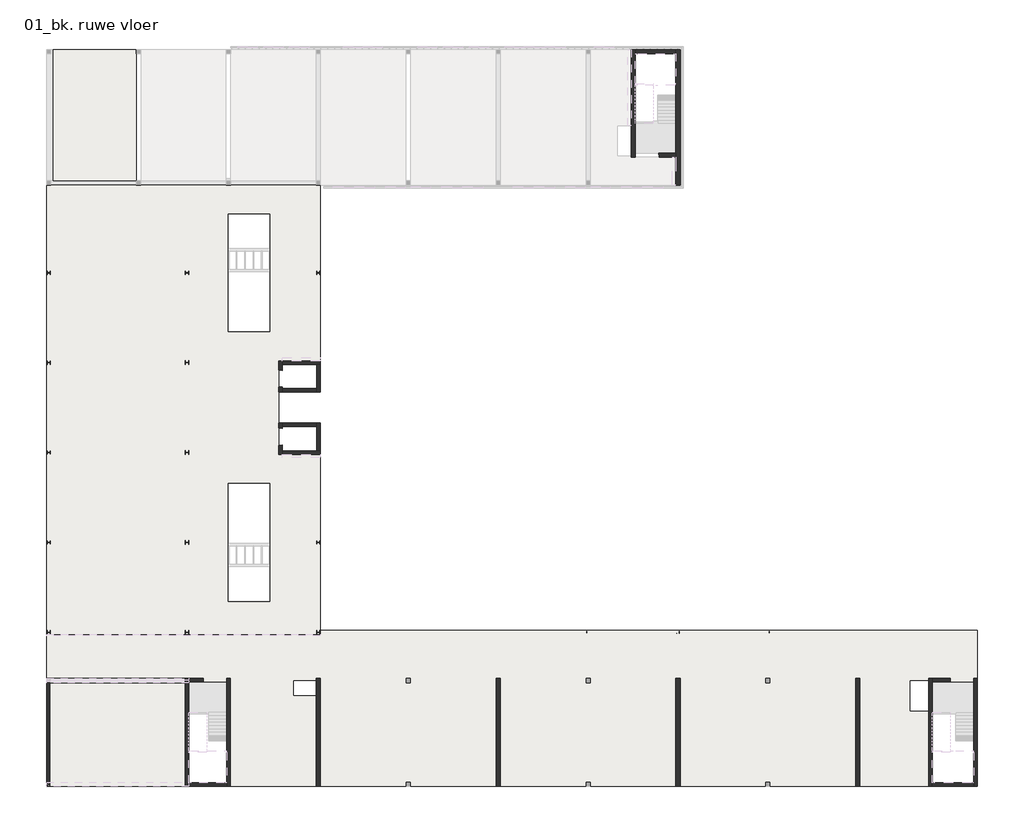
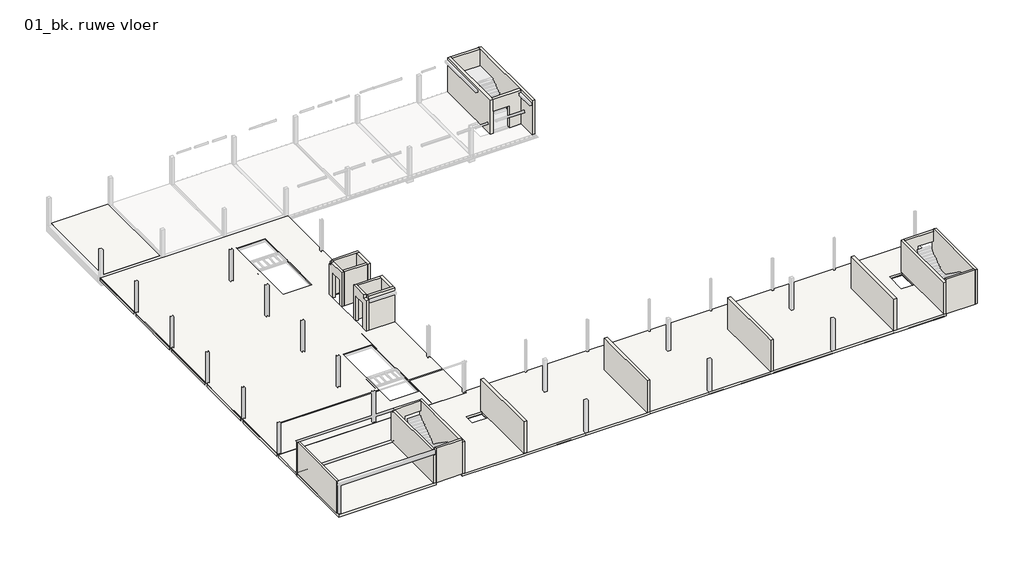
# One storey, part 1 of 4: 25 walls, 20 slabs.
# Revit data of these elements (continued)
# Element 13 (IfcSlab, "NLRS_23_FL_kanaalplaat 260_gen_rsf") (continued)
#   Phase Created = NLRS_nieuw
#   Materials on its faces: "NLRS_f2_beton prefab_gen_rsf"
# Element 14 (IfcSlab, "NLRS_23_FL_kanaalplaat 260_gen_rsf")
#   IfcGUID = "0OswKhMc1Dju7i6LqsCl1d"
#   built-in parameter 1001955 = -1.5708 (stored number, unit not read)
#   Height Offset From Level = -70 mm
#   built-in parameter 1001954 = 1
#   IsExternal = no
#   LoadBearing = yes
#   Phase Created = NLRS_nieuw
#   Materials on its faces: "NLRS_f2_beton prefab_gen_rsf"
# Element 15 (IfcSlab, "NLRS_23_FL_kanaalplaat 260_gen_rsf")
#   IfcGUID = "0OswKhMc1Dju7i6LqsCl1m"
#   Height Offset From Level = -70 mm
#   built-in parameter 1001954 = 1
#   IsExternal = no
#   LoadBearing = yes
#   Phase Created = NLRS_nieuw
#   Materials on its faces: "NLRS_f2_beton prefab_gen_rsf"
# Element 16 (IfcSlab, "NLRS_23_FL_kanaalplaat 260_gen_rsf")
#   IfcGUID = "0OswKhMc1Dju7i6LqsCl2B"
#   built-in parameter 1001955 = 1.5708 (stored number, unit not read)
#   Height Offset From Level = -70 mm
#   built-in parameter 1001954 = 1
#   IsExternal = no
#   LoadBearing = yes
#   Phase Created = NLRS_nieuw
#   Materials on its faces: "NLRS_f2_beton prefab_gen_rsf"
# Element 17 (IfcSlab, "NLRS_23_FL_breedplaat 260_gen_rsf")
#   IfcGUID = "3aMdMHoe12P9KDGPyaIhcT"
#   built-in parameter 1001955 = 1.5708 (stored number, unit not read)
#   Height Offset From Level = 0 mm
#   built-in parameter 1001954 = 1
#   IsExternal = no
#   LoadBearing = yes
#   Phase Created = NLRS_nieuw
#   Materials on its faces: "NLRS_f2_beton ihwg_gen_rsf"
# Element 18 (IfcSlab, "NLRS_23_FL_breedplaat schil 60_gen_rsf")
#   IfcGUID = "2hjDq_lp57$vrUvPCETdlA"
#   Comments = ""
#   built-in parameter 1001955 = -1.5708 (stored number, unit not read)
#   Height Offset From Level = -200 mm
#   built-in parameter 1001954 = 1
#   IsExternal = no
#   LoadBearing = yes
#   Phase Created = NLRS_nieuw
#   Materials on its faces: "NLRS_f2_beton prefab_gen_rsf"
# Element 19 (IfcSlab, "NLRS_23_FL_breedplaat schil 60_gen_rsf")
#   IfcGUID = "2hjDq_lp57$vrUvPCETOIZ"
#   Comments = ""
#   built-in parameter 1001955 = -1.5708 (stored number, unit not read)
#   Height Offset From Level = -200 mm
#   built-in parameter 1001954 = 1
#   IsExternal = no
#   LoadBearing = yes
#   Phase Created = NLRS_nieuw
#   Materials on its faces: "NLRS_f2_beton prefab_gen_rsf"
# Element 20 (IfcSlab, "NLRS_23_FL_breedplaat schil 60_gen_rsf")
#   IfcGUID = "1q3Kx8wcTFnf_3PJz4ij95"
#   Comments = ""
#   Height Offset From Level = -200 mm
#   built-in parameter 1001954 = 1
#   IsExternal = no
#   LoadBearing = yes
#   Phase Created = NLRS_nieuw
#   Materials on its faces: "NLRS_f2_beton prefab_gen_rsf"
# Element 21 (IfcWall, "NLRS_22_WA_beton ihw 250_gen_rsf")
#   IfcGUID = "13lTCcCQ95UOWcvnmPh7qn"
#   Comments = ""
#   Top Offset = 0 mm
#   Base Offset = 0 mm
#   wall height = 3540 mm
#   IsExternal = no
#   LoadBearing = yes
#   Phase Created = NLRS_nieuw
#   Base Constraint = 01_bk. ruwe vloer
#   Top Constraint = 02_ok ruwe vloer
#   Materials on its faces: "NLRS_f2_beton ihwg_gen_rsf"
# Element 22 (IfcWall, "NLRS_22_WA_beton ihw 250_gen_rsf")
#   IfcGUID = "13lTCcCQ95UOWcvnmPh7qi"
#   Comments = ""
#   Top Offset = 0 mm
#   Base Offset = 0 mm
#   wall height = 3540 mm
#   IsExternal = no
#   LoadBearing = yes
#   Phase Created = NLRS_nieuw
#   Base Constraint = 01_bk. ruwe vloer
#   Top Constraint = 02_ok ruwe vloer
#   Materials on its faces: "NLRS_f2_beton ihwg_gen_rsf"
# Element 23 (IfcWall, "NLRS_22_WA_beton ihw 300_gen_rsf")
#   IfcGUID = "13lTCcCQ95UOWcvnmPh7qk"
#   Comments = ""
#   Top Offset = 0 mm
#   Base Offset = 0 mm
#   wall height = 3540 mm
#   IsExternal = no
#   LoadBearing = yes
#   Phase Created = NLRS_nieuw
#   Base Constraint = 01_bk. ruwe vloer
#   Top Constraint = 02_ok ruwe vloer
#   Materials on its faces: "NLRS_f2_beton ihwg_gen_rsf"
# Element 24 (IfcWall, "NLRS_22_WA_beton ihw 300_gen_rsf")
#   IfcGUID = "13lTCcCQ95UOWcvnmPh7qg"
#   Comments = ""
#   Top Offset = 0 mm
#   Base Offset = 0 mm
#   wall height = 3540 mm
#   IsExternal = no
#   LoadBearing = yes
#   Phase Created = NLRS_nieuw
#   Base Constraint = 01_bk. ruwe vloer
#   Top Constraint = 02_ok ruwe vloer
#   Materials on its faces: "NLRS_f2_beton ihwg_gen_rsf"
# Element 25 (IfcWall, "NLRS_22_WA_beton ihw 300_gen_rsf")
#   IfcGUID = "13lTCcCQ95UOWcvnmPh7qc"
#   Comments = ""
#   Top Offset = 0 mm
#   Base Offset = 0 mm
#   wall height = 3540 mm
#   IsExternal = no
#   LoadBearing = yes
#   Phase Created = NLRS_nieuw
#   Base Constraint = 01_bk. ruwe vloer
#   Top Constraint = 02_ok ruwe vloer
#   Materials on its faces: "NLRS_f2_beton ihwg_gen_rsf"
# Element 26 (IfcWall, "NLRS_22_WA_beton ihw 300_gen_rsf")
#   IfcGUID = "13lTCcCQ95UOWcvnmPh7qY"
#   Comments = ""
#   Top Offset = 0 mm
#   Base Offset = 0 mm
#   wall height = 3540 mm
#   IsExternal = no
#   LoadBearing = yes
#   Phase Created = NLRS_nieuw
#   Base Constraint = 01_bk. ruwe vloer
#   Top Constraint = 02_ok ruwe vloer
#   Materials on its faces: "NLRS_f2_beton ihwg_gen_rsf"
# Element 27 (IfcWall, "NLRS_21_WA_beton ihw 250_gen_rsf")
#   IfcGUID = "13lTCcCQ95UOWcvnmPh7rS"
#   Comments = ""
#   Top Offset = 0 mm
#   Base Offset = 0 mm
#   wall height = 3800 mm
#   IsExternal = yes
#   LoadBearing = yes
#   Phase Created = NLRS_nieuw
#   Base Constraint = 01_bk. ruwe vloer
#   Top Constraint = 02_bk ruwe vloer
#   Materials on its faces: "NLRS_f2_beton ihwg_gen_rsf"
# Element 28 (IfcWall, "NLRS_21_WA_kalkzandsteen CS12 214_gen_rsf")
#   IfcGUID = "13lTCcCQ95UOWcvnmPh7rU"
#   Comments = ""
#   Top Offset = 0 mm
#   Base Offset = 0 mm
#   wall height = 3540 mm
#   IsExternal = yes
#   LoadBearing = yes
#   Phase Created = NLRS_nieuw
#   Base Constraint = 01_bk. ruwe vloer
#   Top Constraint = 02_ok ruwe vloer
#   Materials on its faces: "NLRS_f1_kalkzandsteen_gen_rsf"
# Element 29 (IfcWall, "NLRS_21_WA_beton ihw 250_gen_rsf")
#   IfcGUID = "13lTCcCQ95UOWcvnmPh7rO"
#   Top Offset = 0 mm
#   Base Offset = 0 mm
#   wall height = 3800 mm
#   IsExternal = yes
#   LoadBearing = yes
#   Phase Created = NLRS_nieuw
#   Base Constraint = 01_bk. ruwe vloer
#   Top Constraint = 02_bk ruwe vloer
#   Materials on its faces: "NLRS_f2_beton ihwg_gen_rsf"
# Element 30 (IfcWall, "NLRS_22_WA_beton ihw 250_gen_rsf")
#   IfcGUID = "13lTCcCQ95UOWcvnmPh7rQ"
#   Top Offset = 0 mm
#   Base Offset = 0 mm
#   wall height = 3540 mm
#   IsExternal = no
#   LoadBearing = yes
#   Phase Created = NLRS_nieuw
#   Base Constraint = 01_bk. ruwe vloer
#   Top Constraint = 02_ok ruwe vloer
#   Materials on its faces: "NLRS_f2_beton ihwg_gen_rsf"
# Element 31 (IfcWall, "NLRS_22_WA_beton ihw 250_gen_rsf")
#   IfcGUID = "13lTCcCQ95UOWcvnmPh7rK"
#   Comments = ""
#   Top Offset = 0 mm
#   Base Offset = 0 mm
#   wall height = 3540 mm
#   IsExternal = no
#   LoadBearing = yes
#   Phase Created = NLRS_nieuw
#   Base Constraint = 01_bk. ruwe vloer
#   Top Constraint = 02_ok ruwe vloer
#   Materials on its faces: "NLRS_f2_beton ihwg_gen_rsf"
# Element 32 (IfcWall, "NLRS_21_WA_beton ihw 250_gen_rsf")
#   IfcGUID = "13lTCcCQ95UOWcvnmPh7rM"
#   Top Offset = 0 mm
#   Base Offset = 0 mm
#   wall height = 3800 mm
#   IsExternal = yes
#   LoadBearing = yes
#   Phase Created = NLRS_nieuw
#   Base Constraint = 01_bk. ruwe vloer
#   Top Constraint = 02_bk ruwe vloer
#   Materials on its faces: "NLRS_f2_beton ihwg_gen_rsf"
# Element 33 (IfcWall, "NLRS_22_WA_beton ihw 250_gen_rsf")
#   IfcGUID = "13lTCcCQ95UOWcvnmPh7rG"
#   Top Offset = 0 mm
#   Base Offset = 0 mm
#   wall height = 3540 mm
#   IsExternal = no
#   LoadBearing = yes
#   Phase Created = NLRS_nieuw
#   Base Constraint = 01_bk. ruwe vloer
#   Top Constraint = 02_ok ruwe vloer
#   Materials on its faces: "NLRS_f2_beton ihwg_gen_rsf"
# Element 34 (IfcWall, "NLRS_22_WA_beton prefab 300_gen_rsf")
#   IfcGUID = "13lTCcCQ95UOWcvnmPh7s_"
#   Comments = ""
#   built-in parameter 1001111 = 20 mm
#   Top Offset = 0 mm
#   Base Offset = 20 mm
#   wall height = 3780 mm
#   IsExternal = no
#   LoadBearing = yes
#   Phase Created = NLRS_nieuw
#   Base Constraint = 01_bk. ruwe vloer
#   Top Constraint = 02_bk ruwe vloer
#   Materials on its faces: "NLRS_f2_beton prefab_gen_rsf"
# Element 35 (IfcWall, "NLRS_21_WA_beton prefab 300_gen_rsf")
#   IfcGUID = "13lTCcCQ95UOWcvnmPh7sx"
#   Comments = ""
#   built-in parameter 1001111 = 20 mm
#   Top Offset = 0 mm
#   Base Offset = 20 mm
#   wall height = 3780 mm
#   IsExternal = yes
#   LoadBearing = yes
#   Phase Created = NLRS_nieuw
#   Base Constraint = 01_bk. ruwe vloer
#   Top Constraint = 02_bk ruwe vloer
#   Materials on its faces: "NLRS_f2_beton prefab_gen_rsf"
# Element 36 (IfcWall, "NLRS_21_WA_beton prefab 300_gen_rsf")
#   IfcGUID = "13lTCcCQ95UOWcvnmPh7sr"
#   Comments = ""
#   built-in parameter 1001111 = 20 mm
#   Top Offset = 0 mm
#   Base Offset = 20 mm
#   wall height = 3780 mm
#   IsExternal = yes
#   LoadBearing = yes
#   Phase Created = NLRS_nieuw
#   Base Constraint = 01_bk. ruwe vloer
#   Top Constraint = 02_bk ruwe vloer
#   Materials on its faces: "NLRS_f2_beton prefab_gen_rsf"
# Element 37 (IfcWall, "NLRS_22_WA_beton prefab 300_gen_rsf")
#   IfcGUID = "13lTCcCQ95UOWcvnmPh7st"
#   Comments = ""
#   built-in parameter 1001111 = 20 mm
#   Top Offset = 0 mm
#   Base Offset = 20 mm
#   wall height = 3780 mm
#   IsExternal = no
#   LoadBearing = yes
#   Phase Created = NLRS_nieuw
#   Base Constraint = 01_bk. ruwe vloer
#   Top Constraint = 02_bk ruwe vloer
#   Materials on its faces: "NLRS_f2_beton prefab_gen_rsf"
# Element 38 (IfcWall, "NLRS_22_WA_beton prefab 250_gen_rsf")
#   IfcGUID = "13lTCcCQ95UOWcvnmPh7uI"
#   built-in parameter 1001111 = 20 mm
#   Top Offset = 0 mm
#   Base Offset = 20 mm
#   wall height = 3780 mm
#   IsExternal = no
#   LoadBearing = yes
#   Phase Created = NLRS_nieuw
#   Base Constraint = 01_bk. ruwe vloer
#   Top Constraint = 02_bk ruwe vloer
#   Materials on its faces: "NLRS_f2_beton prefab_gen_rsf"
# Element 39 (IfcWall, "NLRS_22_WA_beton prefab 250_gen_rsf")
#   IfcGUID = "13lTCcCQ95UOWcvnmPh7uC"
#   built-in parameter 1001111 = 20 mm
#   Top Offset = 0 mm
#   Base Offset = 20 mm
#   wall height = 3780 mm
#   IsExternal = no
#   LoadBearing = yes
#   Phase Created = NLRS_nieuw
#   Base Constraint = 01_bk. ruwe vloer
#   Top Constraint = 02_bk ruwe vloer
#   Materials on its faces: "NLRS_f2_beton prefab_gen_rsf"
# Element 40 (IfcWall, "NLRS_22_WA_beton prefab 250_gen_rsf")
#   IfcGUID = "13lTCcCQ95UOWcvnmPh7uE"
#   built-in parameter 1001111 = 20 mm
#   Top Offset = 0 mm
#   Base Offset = 20 mm
#   wall height = 3780 mm
#   IsExternal = no
#   LoadBearing = yes
#   Phase Created = NLRS_nieuw
#   Base Constraint = 01_bk. ruwe vloer
#   Top Constraint = 02_bk ruwe vloer
#   Materials on its faces: "NLRS_f2_beton prefab_gen_rsf"
# Element 41 (IfcWall, "NLRS_21_WA_beton prefab 250_gen_rsf")
#   IfcGUID = "13lTCcCQ95UOWcvnmPh7u8"
#   built-in parameter 1001111 = 20 mm
#   Top Offset = 0 mm
#   Base Offset = 20 mm
#   wall height = 3780 mm
#   IsExternal = yes
#   LoadBearing = yes
#   Phase Created = NLRS_nieuw
#   Base Constraint = 01_bk. ruwe vloer
#   Top Constraint = 02_bk ruwe vloer
#   Materials on its faces: "NLRS_f2_beton prefab_gen_rsf"
# Element 42 (IfcWall, "NLRS_22_WA_beton prefab 250_gen_rsf")
#   IfcGUID = "13lTCcCQ95UOWcvnmPh7uA"
#   built-in parameter 1001111 = 20 mm
#   Top Offset = 0 mm
#   Base Offset = 20 mm
#   wall height = 3780 mm
#   IsExternal = no
#   LoadBearing = yes
#   Phase Created = NLRS_nieuw
#   Base Constraint = 01_bk. ruwe vloer
#   Top Constraint = 02_bk ruwe vloer
#   Materials on its faces: "NLRS_f2_beton prefab_gen_rsf"
# Element 43 (IfcWall, "NLRS_22_WA_beton prefab 250_gen_rsf")
#   IfcGUID = "13lTCcCQ95UOWcvnmPh7u4"
#   built-in parameter 1001111 = 20 mm
#   Top Offset = 0 mm
#   Base Offset = 20 mm
#   wall height = 3780 mm
#   IsExternal = no
#   LoadBearing = yes
#   Phase Created = NLRS_nieuw
#   Base Constraint = 01_bk. ruwe vloer
#   Top Constraint = 02_bk ruwe vloer
#   Materials on its faces: "NLRS_f2_beton prefab_gen_rsf"
# Element 44 (IfcWall, "NLRS_22_WA_beton prefab 250_gen_rsf")
#   IfcGUID = "13lTCcCQ95UOWcvnmPh7u6"
#   built-in parameter 1001111 = 20 mm
#   Top Offset = 0 mm
#   Base Offset = 20 mm
#   wall height = 3780 mm
#   IsExternal = no
#   LoadBearing = yes
#   Phase Created = NLRS_nieuw
#   Base Constraint = 01_bk. ruwe vloer
#   Top Constraint = 02_bk ruwe vloer
#   Materials on its faces: "NLRS_f2_beton prefab_gen_rsf"
# Element 45 (IfcWall, "NLRS_21_WA_beton prefab 250_gen_rsf")
#   IfcGUID = "13lTCcCQ95UOWcvnmPh7u0"
#   built-in parameter 1001111 = 20 mm
#   Top Offset = 0 mm
#   Base Offset = 20 mm
#   wall height = 3780 mm
#   IsExternal = yes
#   LoadBearing = yes
#   Phase Created = NLRS_nieuw
#   Base Constraint = 01_bk. ruwe vloer
#   Top Constraint = 02_bk ruwe vloer
#   Materials on its faces: "NLRS_f2_beton prefab_gen_rsf"
# Materials
#   "NLRS_f2_beton ihwg_gen_rsf": class "F - Niet gebakken kunststeen", colour RGB 129 133 118, transparency 0, Keynote = "f2", Manufacturer = "Revit Standards Foundation", URL = "www.revitstandards.org", Description = "beton ihwg", Cost = 0
#   "NLRS_f2_beton prefab_gen_rsf": class "F - Niet gebakken kunststeen", colour RGB 129 133 118, transparency 0, Keynote = "f2", Manufacturer = "Revit Standards Foundation", URL = "www.revitstandards.org", Description = "beton prefab", Cost = 0
#   "NLRS_f1_kalkzandsteen_gen_rsf": class "F - Niet gebakken kunststeen", colour RGB 223 221 219, transparency 0, Keynote = "f1", Manufacturer = "Revit Standards Foundation", URL = "www.revitstandards.org", Description = "kalkzandsteen", Cost = 0
